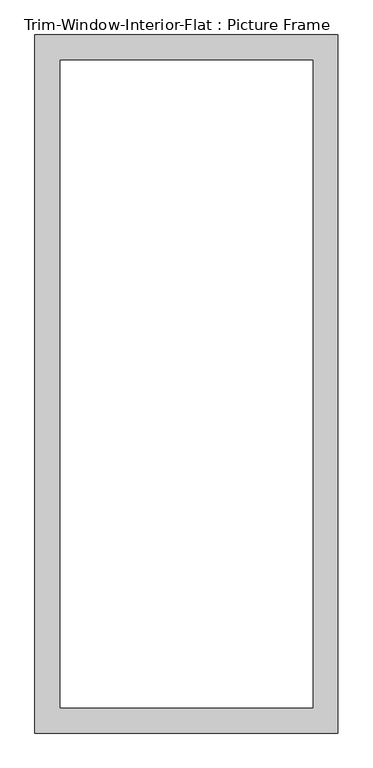
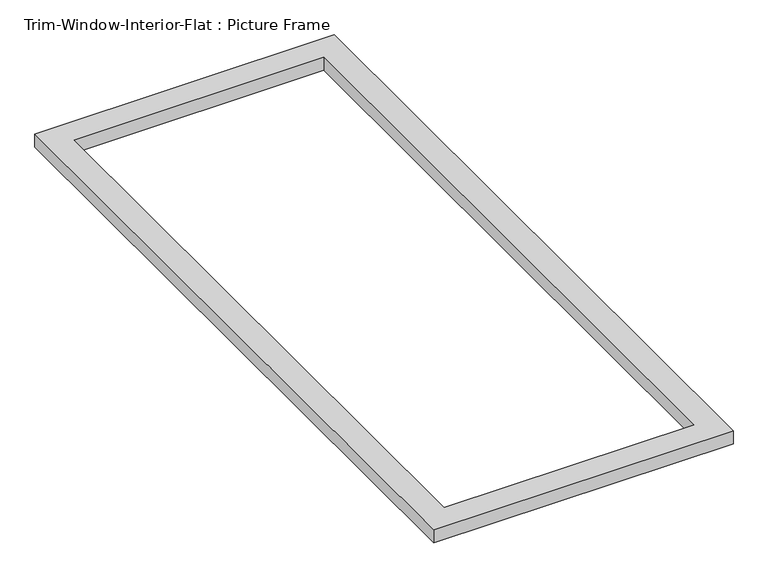
"""IFC4 building model written with IfcOpenShell, lengths in millimetres: proxy geometry, Trim-Window-Interior-Flat : Picture Frame."""

import ifcopenshell
import ifcopenshell.guid

model = None  # the IFC model being written
_history = None  # IfcOwnerHistory: only IFC2X3 demands one
_inside = {}  # id of a spatial element -> (the spatial element, [elements in it])
_under = {}  # id of a project, library or spatial element -> (it, [spatial elements below it])
_declared = {}  # id of a project -> (the project, [libraries it declares])
_typed = {}  # id of a type object -> (the type object, [elements of that type])
_made_of = {}  # id of a material, layer set ... -> (it, [elements and type objects made of it])


def new_model(schema):
    """Start an empty IFC model of exactly this schema.

    Asked for "IFC4X3", IfcOpenShell would pick the latest addendum, in which some entities
    have other attributes; the version numbers below select the first issue.
    IFC2X3 requires an IfcOwnerHistory on every rooted entity: one is made here for all.
    """
    global model, _history
    if schema == "IFC4X3":
        model = ifcopenshell.file(schema_version=(4, 3, 0, 0))
    else:
        model = ifcopenshell.file(schema=schema)
    _inside.clear()
    _under.clear()
    _declared.clear()
    _typed.clear()
    _made_of.clear()
    _history = None
    if model.schema == "IFC2X3":
        org = make("IfcOrganization", Name="unknown")
        user = make(
            "IfcPersonAndOrganization",
            ThePerson=make("IfcPerson", FamilyName="unknown"),
            TheOrganization=org,
        )
        app = make(
            "IfcApplication",
            ApplicationDeveloper=org,
            Version="unknown",
            ApplicationFullName="unknown",
            ApplicationIdentifier="unknown",
        )
        _history = make(
            "IfcOwnerHistory",
            OwningUser=user,
            OwningApplication=app,
            ChangeAction="ADDED",
            CreationDate=0,
        )
    return model


def make(cls, **values):
    """One entity of the class cls with the attributes given. An attribute that is None is left unset."""
    return model.create_entity(
        cls, **{name: value for name, value in values.items() if value is not None}
    )


def rooted(cls, **values):
    """An entity with a GlobalId (a new one), such as an element, a storey or a relation."""
    return make(cls, GlobalId=ifcopenshell.guid.new(), OwnerHistory=_history, **values)


def si_unit(unit_type, name, prefix=None):
    """IfcSIUnit, for example si_unit("LENGTHUNIT", "METRE", prefix="MILLI")."""
    return make("IfcSIUnit", UnitType=unit_type, Prefix=prefix, Name=name)


def assignment(units):
    """IfcUnitAssignment: the units of a project."""
    return None if units is None else make("IfcUnitAssignment", Units=units)


def point(xyz):
    """IfcCartesianPoint."""
    return None if xyz is None else make("IfcCartesianPoint", Coordinates=xyz)


def direction(xyz):
    """IfcDirection."""
    return None if xyz is None else make("IfcDirection", DirectionRatios=xyz)


def frame(location, z_axis=None, x_axis=None):
    """IfcAxis2Placement3D, a coordinate frame: its origin and axes. An axis left out is left unset."""
    return make(
        "IfcAxis2Placement3D",
        Location=point(location),
        Axis=direction(z_axis),
        RefDirection=direction(x_axis),
    )


def origin():
    """The frame at (0, 0, 0) with its axes left unset."""
    return frame((0.0, 0.0, 0.0))


def origin_with_axes():
    """The frame at (0, 0, 0) with the z axis (0, 0, 1) and the x axis (1, 0, 0) written out."""
    return frame((0.0, 0.0, 0.0), z_axis=(0.0, 0.0, 1.0), x_axis=(1.0, 0.0, 0.0))


def place(relative_to, where):
    """IfcLocalPlacement: puts the frame where relative to a parent placement (None: the world)."""
    return make(
        "IfcLocalPlacement", PlacementRelTo=relative_to, RelativePlacement=where
    )


def context(
    kind, dimensions, precision=None, world=None, true_north=None, identifier=None
):
    """IfcGeometricRepresentationContext, for example the 3D "Model" context."""
    return make(
        "IfcGeometricRepresentationContext",
        ContextIdentifier=identifier,
        ContextType=kind,
        CoordinateSpaceDimension=dimensions,
        Precision=precision,
        WorldCoordinateSystem=world,
        TrueNorth=true_north,
    )


def project(units=None, contexts=None):
    """IfcProject with its units and contexts."""
    return rooted(
        "IfcProject",
        Name="project",
        RepresentationContexts=contexts,
        UnitsInContext=assignment(units),
    )


def spatial(cls, under=None, at=None, **own):
    """A site, building, storey or space (cls), placed at a placement, below another one or the project."""
    s = rooted(cls, ObjectPlacement=at, **own)
    if under is not None:
        _under.setdefault(under.id(), (under, []))[1].append(s)
    return s


def polyline(points):
    """IfcPolyline through the points."""
    return make("IfcPolyline", Points=[point(p) for p in points])


def outline(outer, holes=None, kind="AREA"):
    """IfcArbitraryClosedProfileDef: a profile drawn as a closed curve; with holes, ...WithVoids."""
    if holes is None:
        return make("IfcArbitraryClosedProfileDef", ProfileType=kind, OuterCurve=outer)
    return make(
        "IfcArbitraryProfileDefWithVoids",
        ProfileType=kind,
        OuterCurve=outer,
        InnerCurves=holes,
    )


def extrude(swept, where, along, depth):
    """IfcExtrudedAreaSolid: the profile swept, set in the frame where, extruded along a direction by depth."""
    return make(
        "IfcExtrudedAreaSolid",
        SweptArea=swept,
        Position=where,
        ExtrudedDirection=direction(along),
        Depth=depth,
    )


def shape(context_of_items, identifier, shape_type, items):
    """IfcShapeRepresentation: the items that make up one representation, for example the "Body"."""
    return make(
        "IfcShapeRepresentation",
        ContextOfItems=context_of_items,
        RepresentationIdentifier=identifier,
        RepresentationType=shape_type,
        Items=items,
    )


def source(mapping_origin, context_of_items, identifier, shape_type, items):
    """IfcRepresentationMap: a shape defined once, which mapped items show again and again."""
    return make(
        "IfcRepresentationMap",
        MappingOrigin=mapping_origin,
        MappedRepresentation=shape(context_of_items, identifier, shape_type, items),
    )


def transform(
    local_origin,
    x_axis=None,
    y_axis=None,
    z_axis=None,
    scale=None,
    scale2=None,
    scale3=None,
    uniform=True,
):
    """IfcCartesianTransformationOperator3D, or its non-uniform kind. x_axis, y_axis, z_axis: its Axis1, 2, 3."""
    if uniform:
        return make(
            "IfcCartesianTransformationOperator3D",
            Axis1=direction(x_axis),
            Axis2=direction(y_axis),
            LocalOrigin=point(local_origin),
            Scale=scale,
            Axis3=direction(z_axis),
        )
    return make(
        "IfcCartesianTransformationOperator3DnonUniform",
        Axis1=direction(x_axis),
        Axis2=direction(y_axis),
        LocalOrigin=point(local_origin),
        Scale=scale,
        Axis3=direction(z_axis),
        Scale2=scale2,
        Scale3=scale3,
    )


def mapped(mapping_source, mapping_target):
    """IfcMappedItem: shows the shape of a source again, moved by a transform."""
    return make(
        "IfcMappedItem", MappingSource=mapping_source, MappingTarget=mapping_target
    )


def made_of(thing, what):
    """Note that an element or type object is made of a material, layer set ...; save() writes the relation."""
    if what is not None:
        _made_of.setdefault(what.id(), (what, []))[1].append(thing)
    return thing


def element(
    cls,
    number,
    at=None,
    inside=None,
    cuts=None,
    type_object=None,
    material=None,
    context=None,
    identifier="Body",
    shape_type=None,
    held_by="IfcProductDefinitionShape",
    body=None,
    shapes=None,
    **own,
):
    """One element of the class cls, such as IfcWall. Its Tag is "e" and its number.

    at: its placement. inside: the storey or other place that contains it. cuts: it is an
    opening in that element (IfcRelVoidsElement). A single representation is given by context,
    identifier, shape_type and body (its items); several are given by shapes. held_by: the class
    of the entity that holds the representations. save() writes the other relations.
    """
    e = rooted(cls, Tag="e%d" % number, ObjectPlacement=at, **own)
    if body is not None:
        shapes = [shape(context, identifier, shape_type, body)]
    if shapes is not None:
        e.Representation = make(held_by, Representations=shapes)
    if inside is not None:
        _inside.setdefault(inside.id(), (inside, []))[1].append(e)
    if cuts is not None:
        rooted(
            "IfcRelVoidsElement", RelatingBuildingElement=cuts, RelatedOpeningElement=e
        )
    if type_object is not None:
        _typed.setdefault(type_object.id(), (type_object, []))[1].append(e)
    return made_of(e, material)


def aggregate(whole, parts):
    """IfcRelAggregates: a whole, such as a stair, and the parts it consists of."""
    return rooted("IfcRelAggregates", RelatingObject=whole, RelatedObjects=parts)


def save(model, path):
    """Write the relations noted so far, then the file.

    IfcRelAggregates (storeys below a building ...), IfcRelContainedInSpatialStructure (elements
    in a storey), IfcRelDefinesByType, IfcRelAssociatesMaterial and IfcRelDeclares: one each for
    every whole, place, type object, material and project.
    """
    for whole, parts in _under.values():
        aggregate(whole, parts)
    for where, things in _inside.values():
        rooted(
            "IfcRelContainedInSpatialStructure",
            RelatedElements=things,
            RelatingStructure=where,
        )
    for kind, things in _typed.values():
        rooted("IfcRelDefinesByType", RelatedObjects=things, RelatingType=kind)
    for what, things in _made_of.values():
        rooted("IfcRelAssociatesMaterial", RelatedObjects=things, RelatingMaterial=what)
    for by, libraries in _declared.values():
        rooted("IfcRelDeclares", RelatingContext=by, RelatedDefinitions=libraries)
    model.write(path)


def trim_window_interior_flat_picture_frame_5ec1ed24(model_context):
    return source(origin(), model_context, "Body", "SweptSolid", [
        extrude(outline(polyline([(344.45, 44.45), (344.45, -1544.45), (-344.45, -1544.45), (-344.45, 44.45), (344.45, 44.45)]), holes=[polyline([(287.3, -12.7), (-287.3, -12.7), (-287.3, -1487.3), (287.3, -1487.3), (287.3, -12.7)])]), origin_with_axes(), (0.0, 0.0, 1.0), 31.75),
    ])


if __name__ == "__main__":
    model = new_model("IFC4")
    model_context = context("Model", 3, world=origin())
    ifc_project = project(units=[si_unit("LENGTHUNIT", "METRE", prefix="MILLI")], contexts=[model_context])
    site = spatial("IfcSite", under=ifc_project)
    building = spatial("IfcBuilding", under=site)
    placement = place(None, origin())
    trim_window_interior_flat_picture_frame_shape = trim_window_interior_flat_picture_frame_5ec1ed24(model_context)
    element("IfcBuildingElementProxy", 1, Name="Trim-Window-Interior-Flat : Picture Frame", ObjectType="Trim-Window-Interior-Flat : Picture Frame", at=placement, inside=building, context=model_context, shape_type="MappedRepresentation", body=[
        mapped(trim_window_interior_flat_picture_frame_shape, transform((0.0, 0.0, 0.0), x_axis=(1.0, 0.0, 0.0), y_axis=(0.0, 1.0, 0.0), z_axis=(0.0, 0.0, 1.0))),
    ])
    save(model, "model.ifc")

# Revit data of these elements
# Type "Trim-Window-Interior-Flat : Picture Frame"
#   Trim Thickness_Picture Frame = 3.175 cm
#   Trim Width = 5.715 cm
#   Trim Thickness_with Sill = 1.905 cm
#   Sill Thickness = 3.175 cm
#   Opening Width [instance default] = 60.96 cm
#   Opening Height [instance default] = 91.44 cm
#   Default Elevation = 121.92 cm
#   Sill = no
#   Picture Frame = yes
#   Trim Material [instance default] = none
# Element 1 (IfcBuildingElementProxy, "Trim-Window-Interior-Flat : Picture Frame")
#   Opening Width = 60 cm
#   Opening Height = 150 cm
#   Trim Material = Wood - Stained
#   Materials on its faces: "Wood - Stained"
# Materials
#   "Wood - Stained": class "Wood", colour RGB 224 178 126, transparency 0, Cost = 0
